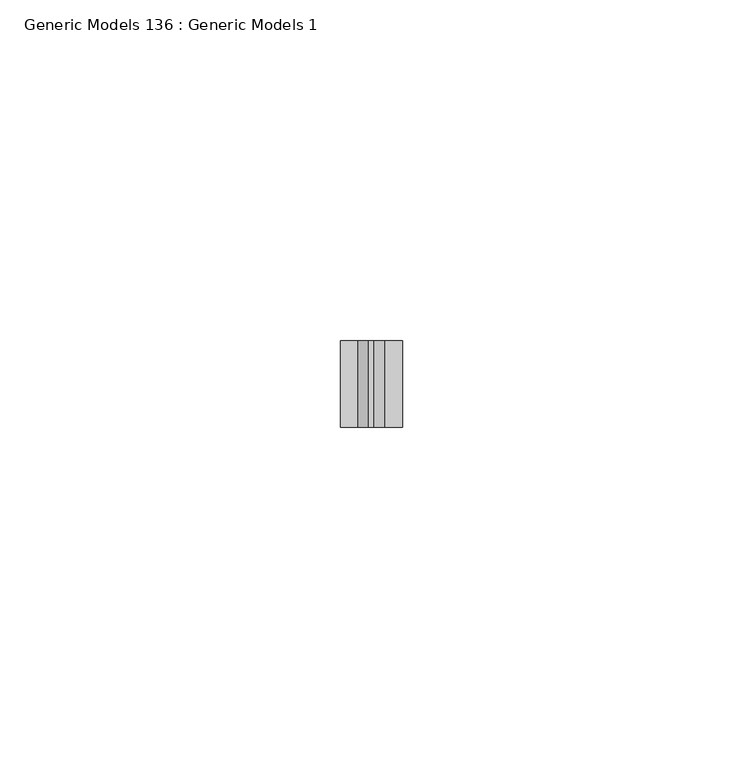
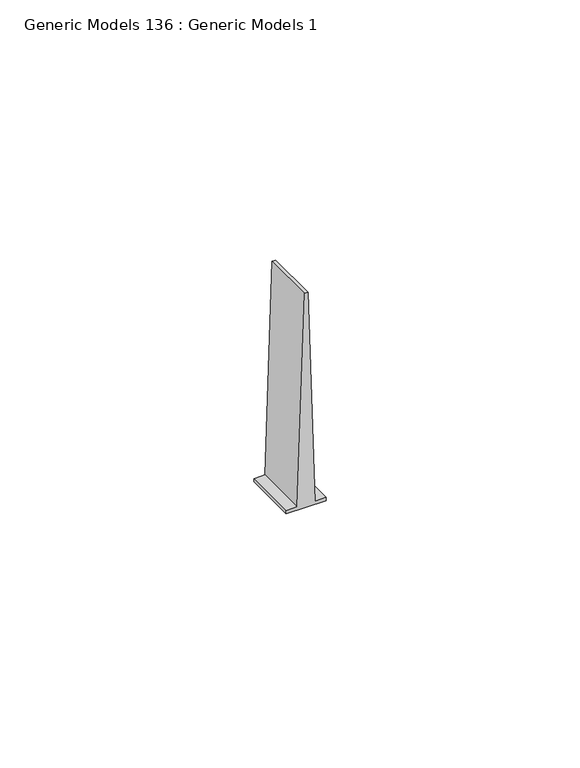
"""IFC4 building model written with IfcOpenShell, lengths in millimetres: proxy geometry, Generic Models 136 : Generic Models 1."""

import ifcopenshell
import ifcopenshell.guid

model = None  # the IFC model being written
_history = None  # IfcOwnerHistory: only IFC2X3 demands one
_inside = {}  # id of a spatial element -> (the spatial element, [elements in it])
_under = {}  # id of a project, library or spatial element -> (it, [spatial elements below it])
_declared = {}  # id of a project -> (the project, [libraries it declares])
_typed = {}  # id of a type object -> (the type object, [elements of that type])
_made_of = {}  # id of a material, layer set ... -> (it, [elements and type objects made of it])


def new_model(schema):
    """Start an empty IFC model of exactly this schema.

    Asked for "IFC4X3", IfcOpenShell would pick the latest addendum, in which some entities
    have other attributes; the version numbers below select the first issue.
    IFC2X3 requires an IfcOwnerHistory on every rooted entity: one is made here for all.
    """
    global model, _history
    if schema == "IFC4X3":
        model = ifcopenshell.file(schema_version=(4, 3, 0, 0))
    else:
        model = ifcopenshell.file(schema=schema)
    _inside.clear()
    _under.clear()
    _declared.clear()
    _typed.clear()
    _made_of.clear()
    _history = None
    if model.schema == "IFC2X3":
        org = make("IfcOrganization", Name="unknown")
        user = make(
            "IfcPersonAndOrganization",
            ThePerson=make("IfcPerson", FamilyName="unknown"),
            TheOrganization=org,
        )
        app = make(
            "IfcApplication",
            ApplicationDeveloper=org,
            Version="unknown",
            ApplicationFullName="unknown",
            ApplicationIdentifier="unknown",
        )
        _history = make(
            "IfcOwnerHistory",
            OwningUser=user,
            OwningApplication=app,
            ChangeAction="ADDED",
            CreationDate=0,
        )
    return model


def make(cls, **values):
    """One entity of the class cls with the attributes given. An attribute that is None is left unset."""
    return model.create_entity(
        cls, **{name: value for name, value in values.items() if value is not None}
    )


def rooted(cls, **values):
    """An entity with a GlobalId (a new one), such as an element, a storey or a relation."""
    return make(cls, GlobalId=ifcopenshell.guid.new(), OwnerHistory=_history, **values)


def si_unit(unit_type, name, prefix=None):
    """IfcSIUnit, for example si_unit("LENGTHUNIT", "METRE", prefix="MILLI")."""
    return make("IfcSIUnit", UnitType=unit_type, Prefix=prefix, Name=name)


def assignment(units):
    """IfcUnitAssignment: the units of a project."""
    return None if units is None else make("IfcUnitAssignment", Units=units)


def point(xyz):
    """IfcCartesianPoint."""
    return None if xyz is None else make("IfcCartesianPoint", Coordinates=xyz)


def direction(xyz):
    """IfcDirection."""
    return None if xyz is None else make("IfcDirection", DirectionRatios=xyz)


def frame(location, z_axis=None, x_axis=None):
    """IfcAxis2Placement3D, a coordinate frame: its origin and axes. An axis left out is left unset."""
    return make(
        "IfcAxis2Placement3D",
        Location=point(location),
        Axis=direction(z_axis),
        RefDirection=direction(x_axis),
    )


def origin():
    """The frame at (0, 0, 0) with its axes left unset."""
    return frame((0.0, 0.0, 0.0))


def place(relative_to, where):
    """IfcLocalPlacement: puts the frame where relative to a parent placement (None: the world)."""
    return make(
        "IfcLocalPlacement", PlacementRelTo=relative_to, RelativePlacement=where
    )


def context(
    kind, dimensions, precision=None, world=None, true_north=None, identifier=None
):
    """IfcGeometricRepresentationContext, for example the 3D "Model" context."""
    return make(
        "IfcGeometricRepresentationContext",
        ContextIdentifier=identifier,
        ContextType=kind,
        CoordinateSpaceDimension=dimensions,
        Precision=precision,
        WorldCoordinateSystem=world,
        TrueNorth=true_north,
    )


def project(units=None, contexts=None):
    """IfcProject with its units and contexts."""
    return rooted(
        "IfcProject",
        Name="project",
        RepresentationContexts=contexts,
        UnitsInContext=assignment(units),
    )


def spatial(cls, under=None, at=None, **own):
    """A site, building, storey or space (cls), placed at a placement, below another one or the project."""
    s = rooted(cls, ObjectPlacement=at, **own)
    if under is not None:
        _under.setdefault(under.id(), (under, []))[1].append(s)
    return s


def polyline(points):
    """IfcPolyline through the points."""
    return make("IfcPolyline", Points=[point(p) for p in points])


def outline(outer, holes=None, kind="AREA"):
    """IfcArbitraryClosedProfileDef: a profile drawn as a closed curve; with holes, ...WithVoids."""
    if holes is None:
        return make("IfcArbitraryClosedProfileDef", ProfileType=kind, OuterCurve=outer)
    return make(
        "IfcArbitraryProfileDefWithVoids",
        ProfileType=kind,
        OuterCurve=outer,
        InnerCurves=holes,
    )


def extrude(swept, where, along, depth):
    """IfcExtrudedAreaSolid: the profile swept, set in the frame where, extruded along a direction by depth."""
    return make(
        "IfcExtrudedAreaSolid",
        SweptArea=swept,
        Position=where,
        ExtrudedDirection=direction(along),
        Depth=depth,
    )


def shape(context_of_items, identifier, shape_type, items):
    """IfcShapeRepresentation: the items that make up one representation, for example the "Body"."""
    return make(
        "IfcShapeRepresentation",
        ContextOfItems=context_of_items,
        RepresentationIdentifier=identifier,
        RepresentationType=shape_type,
        Items=items,
    )


def source(mapping_origin, context_of_items, identifier, shape_type, items):
    """IfcRepresentationMap: a shape defined once, which mapped items show again and again."""
    return make(
        "IfcRepresentationMap",
        MappingOrigin=mapping_origin,
        MappedRepresentation=shape(context_of_items, identifier, shape_type, items),
    )


def transform(
    local_origin,
    x_axis=None,
    y_axis=None,
    z_axis=None,
    scale=None,
    scale2=None,
    scale3=None,
    uniform=True,
):
    """IfcCartesianTransformationOperator3D, or its non-uniform kind. x_axis, y_axis, z_axis: its Axis1, 2, 3."""
    if uniform:
        return make(
            "IfcCartesianTransformationOperator3D",
            Axis1=direction(x_axis),
            Axis2=direction(y_axis),
            LocalOrigin=point(local_origin),
            Scale=scale,
            Axis3=direction(z_axis),
        )
    return make(
        "IfcCartesianTransformationOperator3DnonUniform",
        Axis1=direction(x_axis),
        Axis2=direction(y_axis),
        LocalOrigin=point(local_origin),
        Scale=scale,
        Axis3=direction(z_axis),
        Scale2=scale2,
        Scale3=scale3,
    )


def mapped(mapping_source, mapping_target):
    """IfcMappedItem: shows the shape of a source again, moved by a transform."""
    return make(
        "IfcMappedItem", MappingSource=mapping_source, MappingTarget=mapping_target
    )


def made_of(thing, what):
    """Note that an element or type object is made of a material, layer set ...; save() writes the relation."""
    if what is not None:
        _made_of.setdefault(what.id(), (what, []))[1].append(thing)
    return thing


def element(
    cls,
    number,
    at=None,
    inside=None,
    cuts=None,
    type_object=None,
    material=None,
    context=None,
    identifier="Body",
    shape_type=None,
    held_by="IfcProductDefinitionShape",
    body=None,
    shapes=None,
    **own,
):
    """One element of the class cls, such as IfcWall. Its Tag is "e" and its number.

    at: its placement. inside: the storey or other place that contains it. cuts: it is an
    opening in that element (IfcRelVoidsElement). A single representation is given by context,
    identifier, shape_type and body (its items); several are given by shapes. held_by: the class
    of the entity that holds the representations. save() writes the other relations.
    """
    e = rooted(cls, Tag="e%d" % number, ObjectPlacement=at, **own)
    if body is not None:
        shapes = [shape(context, identifier, shape_type, body)]
    if shapes is not None:
        e.Representation = make(held_by, Representations=shapes)
    if inside is not None:
        _inside.setdefault(inside.id(), (inside, []))[1].append(e)
    if cuts is not None:
        rooted(
            "IfcRelVoidsElement", RelatingBuildingElement=cuts, RelatedOpeningElement=e
        )
    if type_object is not None:
        _typed.setdefault(type_object.id(), (type_object, []))[1].append(e)
    return made_of(e, material)


def aggregate(whole, parts):
    """IfcRelAggregates: a whole, such as a stair, and the parts it consists of."""
    return rooted("IfcRelAggregates", RelatingObject=whole, RelatedObjects=parts)


def save(model, path):
    """Write the relations noted so far, then the file.

    IfcRelAggregates (storeys below a building ...), IfcRelContainedInSpatialStructure (elements
    in a storey), IfcRelDefinesByType, IfcRelAssociatesMaterial and IfcRelDeclares: one each for
    every whole, place, type object, material and project.
    """
    for whole, parts in _under.values():
        aggregate(whole, parts)
    for where, things in _inside.values():
        rooted(
            "IfcRelContainedInSpatialStructure",
            RelatedElements=things,
            RelatingStructure=where,
        )
    for kind, things in _typed.values():
        rooted("IfcRelDefinesByType", RelatedObjects=things, RelatingType=kind)
    for what, things in _made_of.values():
        rooted("IfcRelAssociatesMaterial", RelatedObjects=things, RelatingMaterial=what)
    for by, libraries in _declared.values():
        rooted("IfcRelDeclares", RelatingContext=by, RelatedDefinitions=libraries)
    model.write(path)


def generic_models_136_generic_models_1_7576d418(model_context):
    return source(origin(), model_context, "Body", "SweptSolid", [
        extrude(outline(polyline([(2229.092683, 46885.2894531), (2229.092683, 46894.3826531), (2229.886433, 46894.3826531), (2229.886433, 46891.8327895), (2280.686433, 46890.2354003), (2280.686433, 46889.4367058), (2229.886433, 46887.8393167), (2229.886433, 46885.2894531), (2229.092683, 46885.2894531)])), frame((0.0, 565.15, 0.0), z_axis=(0.0, 1.0, 0.0), x_axis=(0.0, 0.0, 1.0)), (0.0, 0.0, 1.0), 12.7),
    ])


if __name__ == "__main__":
    model = new_model("IFC4")
    model_context = context("Model", 3, world=origin())
    ifc_project = project(units=[si_unit("LENGTHUNIT", "METRE", prefix="MILLI")], contexts=[model_context])
    site = spatial("IfcSite", under=ifc_project)
    building = spatial("IfcBuilding", under=site)
    placement = place(None, origin())
    generic_models_136_generic_models_1_shape = generic_models_136_generic_models_1_7576d418(model_context)
    element("IfcBuildingElementProxy", 1, Name="Generic Models 136 : Generic Models 1", ObjectType="Generic Models 136 : Generic Models 1", at=placement, inside=building, context=model_context, shape_type="MappedRepresentation", body=[
        mapped(generic_models_136_generic_models_1_shape, transform((0.0, 0.0, 0.0), x_axis=(1.0, 0.0, 0.0), y_axis=(0.0, 1.0, 0.0), z_axis=(0.0, 0.0, 1.0))),
    ])
    save(model, "model.ifc")

# Revit data of these elements
# Element 1 (IfcBuildingElementProxy, "Generic Models 136 : Generic Models 1")
#   Materials on its faces: "METAL RUNNER CHANNEL; FASTEN @ 24\" O.C."
# Materials
#   "METAL RUNNER CHANNEL; FASTEN @ 24\" O.C.": class "Unassigned", colour RGB 210 209 208, transparency 0, Keynote = "M05121300.02", Cost = 0
